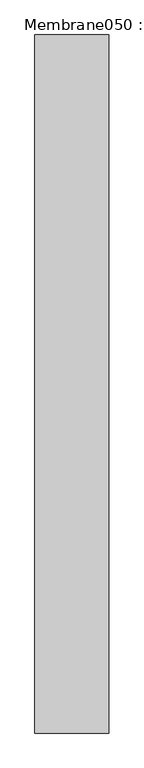
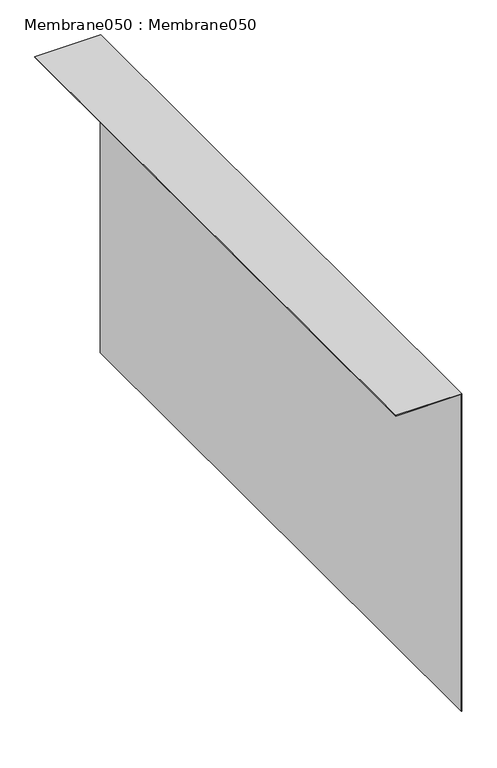
"""IFC4 building model written with IfcOpenShell, lengths in millimetres: proxy geometry, Membrane050 : Membrane050."""

from ifc_helpers import new_model, si_unit, frame, origin, place, context, project, spatial, polyline, outline, extrude, source, transform, mapped, element, save


def membrane050_membrane050_7573ebd2(model_context):
    return source(origin(), model_context, "Body", "SweptSolid", [
        extrude(outline(polyline([(33387.09375, -10092.3525391), (32314.8961275, -10092.3525391), (32314.8961275, -10090.3525391), (33389.09375, -10090.3525391), (33389.09375, -10301.6737014), (33387.09375, -10301.6737014), (33387.09375, -10092.3525391)])), frame((0.0, 7182.1531721, 0.0), z_axis=(0.0, 1.0, 0.0), x_axis=(0.0, 0.0, 1.0)), (0.0, 0.0, 1.0), 2000.0),
    ])


if __name__ == "__main__":
    model = new_model("IFC4")
    model_context = context("Model", 3, world=origin())
    ifc_project = project(units=[si_unit("LENGTHUNIT", "METRE", prefix="MILLI")], contexts=[model_context])
    site = spatial("IfcSite", under=ifc_project)
    building = spatial("IfcBuilding", under=site)
    placement = place(None, origin())
    membrane050_membrane050_shape = membrane050_membrane050_7573ebd2(model_context)
    element("IfcBuildingElementProxy", 1, Name="Membrane050 : Membrane050", ObjectType="Membrane050 : Membrane050", at=placement, inside=building, context=model_context, shape_type="MappedRepresentation", body=[
        mapped(membrane050_membrane050_shape, transform((0.0, 0.0, 0.0), x_axis=(1.0, 0.0, 0.0), y_axis=(0.0, 1.0, 0.0), z_axis=(0.0, 0.0, 1.0))),
    ])
    save(model, "model.ifc")

# Revit data of these elements
# Type "Membrane050 : Membrane050"
#   NameOverride = "Membrane050"
# Element 1 (IfcBuildingElementProxy, "Membrane050 : Membrane050")
#   Materials on its faces: "BITUMINOUS MEMBRANE"
# Materials
#   "BITUMINOUS MEMBRANE": class "Unassigned", colour RGB 0 171 31, transparency 0, Cost = 0
